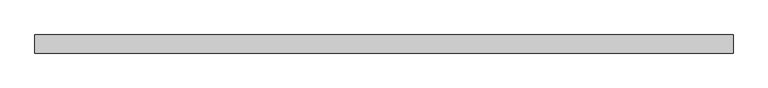
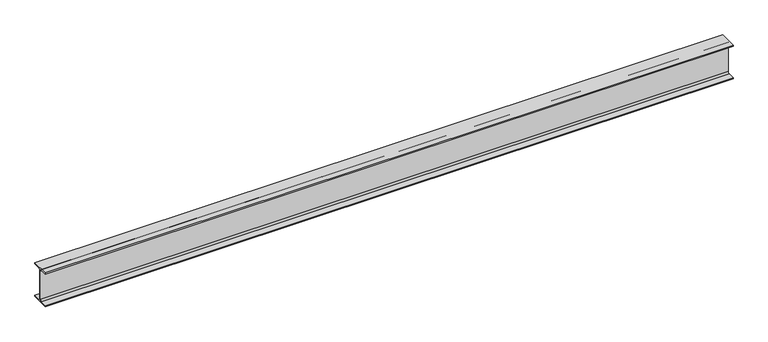
"""IFC4 building model written with IfcOpenShell, lengths in millimetres: beam geometry, 0912_Steel Framing_H-KSD3502 : H_SB_ASB_H-250x125x6x9."""

from ifc_helpers import new_model, si_unit, point, frame, frame_2d, origin, place, context, project, spatial, polyline, circle_curve, trimmed, segment, composite_curve, outline, extrude, source, transform, mapped, element, save


def beam_ce281c4f(model_context):
    return source(origin(), model_context, "Body", "SweptSolid", [
        extrude(outline(composite_curve([segment(polyline([(62.5, -116.0), (62.5, -125.0), (-62.5, -125.0), (-62.5, -116.0), (-15.0, -116.0)]), True, "CONTINUOUS"), segment(trimmed(circle_curve(frame_2d((-15.0, -104.0)), 12.0), [point((-15.0, -116.0))], [point((-3.0, -104.0))], True, "CARTESIAN"), True, "CONTINUOUS"), segment(polyline([(-3.0, -104.0), (-3.0, 104.0)]), True, "CONTINUOUS"), segment(trimmed(circle_curve(frame_2d((-15.0, 104.0)), 12.0), [point((-3.0, 104.0))], [point((-15.0, 116.0))], True, "CARTESIAN"), True, "CONTINUOUS"), segment(polyline([(-15.0, 116.0), (-62.5, 116.0), (-62.5, 125.0), (62.5, 125.0), (62.5, 116.0), (15.0, 116.0)]), True, "CONTINUOUS"), segment(trimmed(circle_curve(frame_2d((15.0, 104.0)), 12.0), [point((15.0, 116.0))], [point((3.0, 104.0))], True, "CARTESIAN"), True, "CONTINUOUS"), segment(polyline([(3.0, 104.0), (3.0, -104.0)]), True, "CONTINUOUS"), segment(trimmed(circle_curve(frame_2d((15.0, -104.0)), 12.0), [point((3.0, -104.0))], [point((15.0, -116.0))], True, "CARTESIAN"), True, "CONTINUOUS"), segment(polyline([(15.0, -116.0), (62.5, -116.0)]), True, "CONTINUOUS")], self_intersect=False)), frame((-2403.3634808, 0.0, 0.0), z_axis=(1.0, 0.0, 0.0), x_axis=(0.0, 1.0, 0.0)), (0.0, 0.0, 1.0), 4815.6934866),
    ])


if __name__ == "__main__":
    model = new_model("IFC4")
    model_context = context("Model", 3, world=origin())
    ifc_project = project(units=[si_unit("LENGTHUNIT", "METRE", prefix="MILLI")], contexts=[model_context])
    site = spatial("IfcSite", under=ifc_project)
    building = spatial("IfcBuilding", under=site)
    placement = place(None, origin())
    beam_shape = beam_ce281c4f(model_context)
    element("IfcBeam", 1, ObjectType="0912_Steel Framing_H-KSD3502 : H_SB_ASB_H-250x125x6x9", at=placement, inside=building, context=model_context, shape_type="MappedRepresentation", body=[
        mapped(beam_shape, transform((0.0, 0.0, 0.0), x_axis=(1.0, 0.0, 0.0), y_axis=(0.0, 1.0, 0.0), z_axis=(0.0, 0.0, 1.0))),
    ])
    save(model, "model.ifc")

# Revit data of these elements
# Type "0912_Steel Framing_H-KSD3502 : H_SB_ASB_H-250x125x6x9"
#   H_WM Code_1 = "S01AA003-00001 | Main Steel Structure Fabrication Work | Shelter/Building | Light Steel - Standard (30KG/M>Weight) | Material: (   )"
#   H_WM Code_2 = "S03AA029-00001 | Main Steel Structure Erection Work | Shelter/Building | Light Steel (30KG/M>Weight) | Material: (   )"
#   H_WM Code_3 = "S01AA010-00001 | Main Steel Structure Fabrication Work | Shelter/Building | Steel Painting/Coating | for Non-Fireproofed Steel Surface, Surface Preparation, Primer, Second & Final Coat | Material: (   )"
#   H_Q'ty Cal Type Tag = "SB-Q2"
#   Width = 12.5 cm
#   Web Thickness = 0.6 cm
#   Web Fillet = 1.2 cm
#   Warping Constant = 42539.8 cm⁶
#   W = 0
#   Torsional Moment of Inertia = 7.8102 cm⁴
#   Section Area = 37.66 cm²
#   Plastic Modulus weak axis = 73.1 cm³
#   Plastic Modulus strong axis = 366.0 cm³
#   Perimeter = 0.97 m²/m
#   Nominal Weight = 29.60 kgf/m
#   Moment of Inertia weak axis = 294.00 cm⁴
#   Moment of Inertia strong axis = 4050.00 cm⁴
#   Height = 25.0 cm
#   Flange Thickness = 0.9 cm
#   Elastic Modulus weak axis = 47.0 cm³
#   Elastic Modulus strong axis = 324.0 cm³
#   Centroid Vertical = 12.5 cm
#   Centroid Horizontal = 6.25 cm
#   Ix = 40500000
#   Length [instance default] = 1.5240 m
#   Zx = 366000
#   b = 0.1250 m
#   h = 0.2500 m
#   r = 0.0120 m
#   s = 0.0060 m
#   t = 0.0090 m
#   A = 0.003766 m²
#   Structural Material [instance default] = Steel, 45-345
#   Assembly Code = ""
# Element 1 (IfcBeam, "0912_Steel Framing_H-KSD3502 : H_SB_ASB_H-250x125x6x9")
#   Structural Material = none
# Materials
#   "Steel, 45-345": class "Metal", colour RGB 189 187 185, transparency 0, Description = "Steel 345 MPa", Cost = 0
